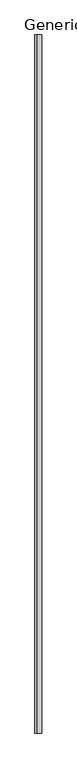
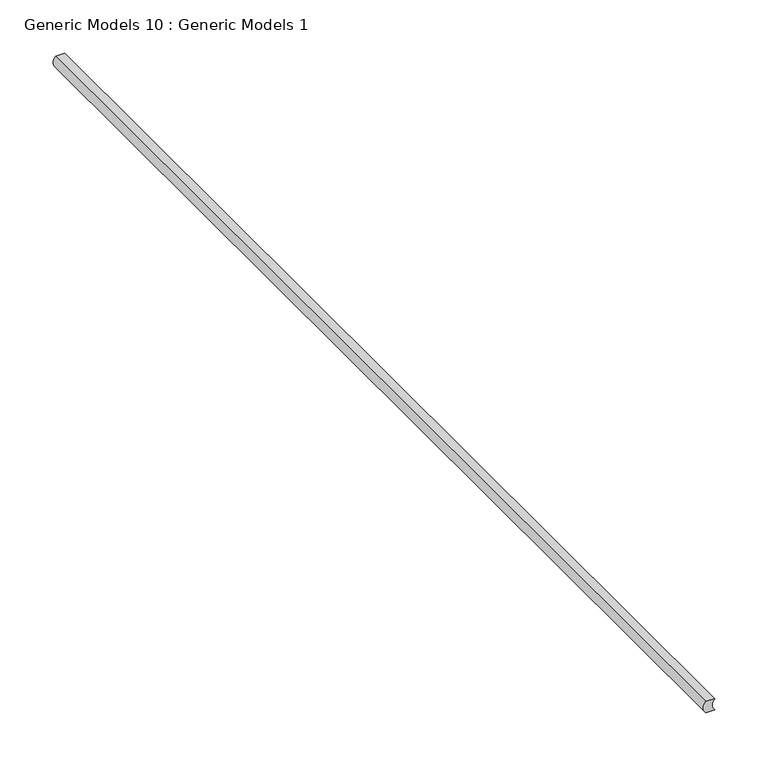
"""IFC4 building model written with IfcOpenShell, lengths in millimetres: proxy geometry, Generic Models 10 : Generic Models 1."""

import ifcopenshell
import ifcopenshell.guid

model = None  # the IFC model being written
_history = None  # IfcOwnerHistory: only IFC2X3 demands one
_inside = {}  # id of a spatial element -> (the spatial element, [elements in it])
_under = {}  # id of a project, library or spatial element -> (it, [spatial elements below it])
_declared = {}  # id of a project -> (the project, [libraries it declares])
_typed = {}  # id of a type object -> (the type object, [elements of that type])
_made_of = {}  # id of a material, layer set ... -> (it, [elements and type objects made of it])


def new_model(schema):
    """Start an empty IFC model of exactly this schema.

    Asked for "IFC4X3", IfcOpenShell would pick the latest addendum, in which some entities
    have other attributes; the version numbers below select the first issue.
    IFC2X3 requires an IfcOwnerHistory on every rooted entity: one is made here for all.
    """
    global model, _history
    if schema == "IFC4X3":
        model = ifcopenshell.file(schema_version=(4, 3, 0, 0))
    else:
        model = ifcopenshell.file(schema=schema)
    _inside.clear()
    _under.clear()
    _declared.clear()
    _typed.clear()
    _made_of.clear()
    _history = None
    if model.schema == "IFC2X3":
        org = make("IfcOrganization", Name="unknown")
        user = make(
            "IfcPersonAndOrganization",
            ThePerson=make("IfcPerson", FamilyName="unknown"),
            TheOrganization=org,
        )
        app = make(
            "IfcApplication",
            ApplicationDeveloper=org,
            Version="unknown",
            ApplicationFullName="unknown",
            ApplicationIdentifier="unknown",
        )
        _history = make(
            "IfcOwnerHistory",
            OwningUser=user,
            OwningApplication=app,
            ChangeAction="ADDED",
            CreationDate=0,
        )
    return model


def make(cls, **values):
    """One entity of the class cls with the attributes given. An attribute that is None is left unset."""
    return model.create_entity(
        cls, **{name: value for name, value in values.items() if value is not None}
    )


def rooted(cls, **values):
    """An entity with a GlobalId (a new one), such as an element, a storey or a relation."""
    return make(cls, GlobalId=ifcopenshell.guid.new(), OwnerHistory=_history, **values)


def si_unit(unit_type, name, prefix=None):
    """IfcSIUnit, for example si_unit("LENGTHUNIT", "METRE", prefix="MILLI")."""
    return make("IfcSIUnit", UnitType=unit_type, Prefix=prefix, Name=name)


def assignment(units):
    """IfcUnitAssignment: the units of a project."""
    return None if units is None else make("IfcUnitAssignment", Units=units)


def point(xyz):
    """IfcCartesianPoint."""
    return None if xyz is None else make("IfcCartesianPoint", Coordinates=xyz)


def direction(xyz):
    """IfcDirection."""
    return None if xyz is None else make("IfcDirection", DirectionRatios=xyz)


def frame(location, z_axis=None, x_axis=None):
    """IfcAxis2Placement3D, a coordinate frame: its origin and axes. An axis left out is left unset."""
    return make(
        "IfcAxis2Placement3D",
        Location=point(location),
        Axis=direction(z_axis),
        RefDirection=direction(x_axis),
    )


def frame_2d(location, x_axis=None):
    """IfcAxis2Placement2D, a coordinate frame in the plane: its origin and x axis."""
    return make(
        "IfcAxis2Placement2D", Location=point(location), RefDirection=direction(x_axis)
    )


def origin():
    """The frame at (0, 0, 0) with its axes left unset."""
    return frame((0.0, 0.0, 0.0))


def place(relative_to, where):
    """IfcLocalPlacement: puts the frame where relative to a parent placement (None: the world)."""
    return make(
        "IfcLocalPlacement", PlacementRelTo=relative_to, RelativePlacement=where
    )


def context(
    kind, dimensions, precision=None, world=None, true_north=None, identifier=None
):
    """IfcGeometricRepresentationContext, for example the 3D "Model" context."""
    return make(
        "IfcGeometricRepresentationContext",
        ContextIdentifier=identifier,
        ContextType=kind,
        CoordinateSpaceDimension=dimensions,
        Precision=precision,
        WorldCoordinateSystem=world,
        TrueNorth=true_north,
    )


def project(units=None, contexts=None):
    """IfcProject with its units and contexts."""
    return rooted(
        "IfcProject",
        Name="project",
        RepresentationContexts=contexts,
        UnitsInContext=assignment(units),
    )


def spatial(cls, under=None, at=None, **own):
    """A site, building, storey or space (cls), placed at a placement, below another one or the project."""
    s = rooted(cls, ObjectPlacement=at, **own)
    if under is not None:
        _under.setdefault(under.id(), (under, []))[1].append(s)
    return s


def polyline(points):
    """IfcPolyline through the points."""
    return make("IfcPolyline", Points=[point(p) for p in points])


def circle_curve(where, radius):
    """IfcCircle in the frame where."""
    return make("IfcCircle", Position=where, Radius=radius)


def trimmed(basis, trim1, trim2, sense, master):
    """IfcTrimmedCurve: the piece of a basis curve between two trims."""
    return make(
        "IfcTrimmedCurve",
        BasisCurve=basis,
        Trim1=trim1,
        Trim2=trim2,
        SenseAgreement=sense,
        MasterRepresentation=master,
    )


def segment(curve, same_sense, transition):
    """IfcCompositeCurveSegment."""
    return make(
        "IfcCompositeCurveSegment",
        Transition=transition,
        SameSense=same_sense,
        ParentCurve=curve,
    )


def composite_curve(segments, self_intersect=None):
    """IfcCompositeCurve: segments joined end to end."""
    return make("IfcCompositeCurve", Segments=segments, SelfIntersect=self_intersect)


def outline(outer, holes=None, kind="AREA"):
    """IfcArbitraryClosedProfileDef: a profile drawn as a closed curve; with holes, ...WithVoids."""
    if holes is None:
        return make("IfcArbitraryClosedProfileDef", ProfileType=kind, OuterCurve=outer)
    return make(
        "IfcArbitraryProfileDefWithVoids",
        ProfileType=kind,
        OuterCurve=outer,
        InnerCurves=holes,
    )


def extrude(swept, where, along, depth):
    """IfcExtrudedAreaSolid: the profile swept, set in the frame where, extruded along a direction by depth."""
    return make(
        "IfcExtrudedAreaSolid",
        SweptArea=swept,
        Position=where,
        ExtrudedDirection=direction(along),
        Depth=depth,
    )


def shape(context_of_items, identifier, shape_type, items):
    """IfcShapeRepresentation: the items that make up one representation, for example the "Body"."""
    return make(
        "IfcShapeRepresentation",
        ContextOfItems=context_of_items,
        RepresentationIdentifier=identifier,
        RepresentationType=shape_type,
        Items=items,
    )


def source(mapping_origin, context_of_items, identifier, shape_type, items):
    """IfcRepresentationMap: a shape defined once, which mapped items show again and again."""
    return make(
        "IfcRepresentationMap",
        MappingOrigin=mapping_origin,
        MappedRepresentation=shape(context_of_items, identifier, shape_type, items),
    )


def transform(
    local_origin,
    x_axis=None,
    y_axis=None,
    z_axis=None,
    scale=None,
    scale2=None,
    scale3=None,
    uniform=True,
):
    """IfcCartesianTransformationOperator3D, or its non-uniform kind. x_axis, y_axis, z_axis: its Axis1, 2, 3."""
    if uniform:
        return make(
            "IfcCartesianTransformationOperator3D",
            Axis1=direction(x_axis),
            Axis2=direction(y_axis),
            LocalOrigin=point(local_origin),
            Scale=scale,
            Axis3=direction(z_axis),
        )
    return make(
        "IfcCartesianTransformationOperator3DnonUniform",
        Axis1=direction(x_axis),
        Axis2=direction(y_axis),
        LocalOrigin=point(local_origin),
        Scale=scale,
        Axis3=direction(z_axis),
        Scale2=scale2,
        Scale3=scale3,
    )


def mapped(mapping_source, mapping_target):
    """IfcMappedItem: shows the shape of a source again, moved by a transform."""
    return make(
        "IfcMappedItem", MappingSource=mapping_source, MappingTarget=mapping_target
    )


def made_of(thing, what):
    """Note that an element or type object is made of a material, layer set ...; save() writes the relation."""
    if what is not None:
        _made_of.setdefault(what.id(), (what, []))[1].append(thing)
    return thing


def element(
    cls,
    number,
    at=None,
    inside=None,
    cuts=None,
    type_object=None,
    material=None,
    context=None,
    identifier="Body",
    shape_type=None,
    held_by="IfcProductDefinitionShape",
    body=None,
    shapes=None,
    **own,
):
    """One element of the class cls, such as IfcWall. Its Tag is "e" and its number.

    at: its placement. inside: the storey or other place that contains it. cuts: it is an
    opening in that element (IfcRelVoidsElement). A single representation is given by context,
    identifier, shape_type and body (its items); several are given by shapes. held_by: the class
    of the entity that holds the representations. save() writes the other relations.
    """
    e = rooted(cls, Tag="e%d" % number, ObjectPlacement=at, **own)
    if body is not None:
        shapes = [shape(context, identifier, shape_type, body)]
    if shapes is not None:
        e.Representation = make(held_by, Representations=shapes)
    if inside is not None:
        _inside.setdefault(inside.id(), (inside, []))[1].append(e)
    if cuts is not None:
        rooted(
            "IfcRelVoidsElement", RelatingBuildingElement=cuts, RelatedOpeningElement=e
        )
    if type_object is not None:
        _typed.setdefault(type_object.id(), (type_object, []))[1].append(e)
    return made_of(e, material)


def aggregate(whole, parts):
    """IfcRelAggregates: a whole, such as a stair, and the parts it consists of."""
    return rooted("IfcRelAggregates", RelatingObject=whole, RelatedObjects=parts)


def save(model, path):
    """Write the relations noted so far, then the file.

    IfcRelAggregates (storeys below a building ...), IfcRelContainedInSpatialStructure (elements
    in a storey), IfcRelDefinesByType, IfcRelAssociatesMaterial and IfcRelDeclares: one each for
    every whole, place, type object, material and project.
    """
    for whole, parts in _under.values():
        aggregate(whole, parts)
    for where, things in _inside.values():
        rooted(
            "IfcRelContainedInSpatialStructure",
            RelatedElements=things,
            RelatingStructure=where,
        )
    for kind, things in _typed.values():
        rooted("IfcRelDefinesByType", RelatedObjects=things, RelatingType=kind)
    for what, things in _made_of.values():
        rooted("IfcRelAssociatesMaterial", RelatedObjects=things, RelatingMaterial=what)
    for by, libraries in _declared.values():
        rooted("IfcRelDeclares", RelatingContext=by, RelatedDefinitions=libraries)
    model.write(path)


def generic_models_10_generic_models_1_db778090(model_context):
    return source(origin(), model_context, "Body", "SweptSolid", [
        extrude(outline(composite_curve([segment(trimmed(circle_curve(frame_2d((2444.75, 51037.604481)), 8.620055), [point((2438.4, 51031.775))], [point((2451.1, 51031.775))], True, "CARTESIAN"), True, "CONTINUOUS"), segment(polyline([(2451.1, 51031.775), (2451.1, 51022.25)]), True, "CONTINUOUS"), segment(trimmed(circle_curve(frame_2d((2444.75, 51028.079481)), 8.620055), [point((2451.1, 51022.25))], [point((2438.4, 51022.25))], False, "CARTESIAN"), True, "CONTINUOUS"), segment(polyline([(2438.4, 51022.25), (2438.4, 51031.775)]), True, "CONTINUOUS")], self_intersect=False)), frame((0.0, 0.0, 0.0), z_axis=(0.0, 1.0, 0.0), x_axis=(0.0, 0.0, 1.0)), (0.0, 0.0, 1.0), 1219.2),
    ])


if __name__ == "__main__":
    model = new_model("IFC4")
    model_context = context("Model", 3, world=origin())
    ifc_project = project(units=[si_unit("LENGTHUNIT", "METRE", prefix="MILLI")], contexts=[model_context])
    site = spatial("IfcSite", under=ifc_project)
    building = spatial("IfcBuilding", under=site)
    placement = place(None, origin())
    generic_models_10_generic_models_1_shape = generic_models_10_generic_models_1_db778090(model_context)
    element("IfcBuildingElementProxy", 1, Name="Generic Models 10 : Generic Models 1", ObjectType="Generic Models 10 : Generic Models 1", at=placement, inside=building, context=model_context, shape_type="MappedRepresentation", body=[
        mapped(generic_models_10_generic_models_1_shape, transform((0.0, 0.0, 0.0), x_axis=(1.0, 0.0, 0.0), y_axis=(0.0, 1.0, 0.0), z_axis=(0.0, 0.0, 1.0))),
    ])
    save(model, "model.ifc")

# Revit data of these elements
# Element 1 (IfcBuildingElementProxy, "Generic Models 10 : Generic Models 1")
#   Materials on its faces: "ACOUSTICAL SEALANT"
# Materials
#   "ACOUSTICAL SEALANT": class "Unassigned", colour RGB 120 120 120, transparency 0, Cost = 0
